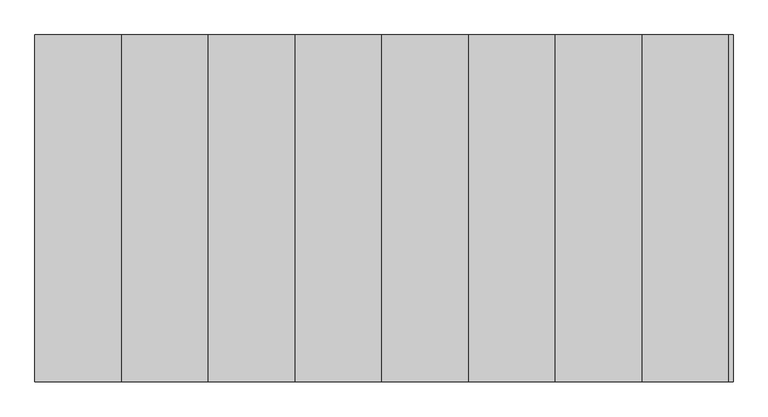
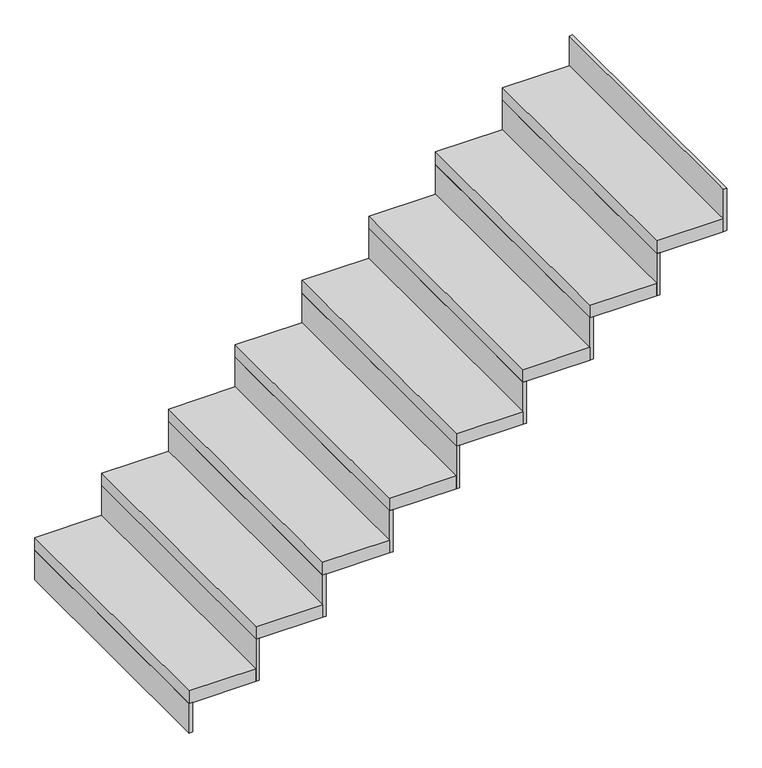
"""IFC4 building model written with IfcOpenShell, lengths in millimetres: stair flight geometry."""

import ifcopenshell
import ifcopenshell.guid

model = None  # the IFC model being written
_history = None  # IfcOwnerHistory: only IFC2X3 demands one
_inside = {}  # id of a spatial element -> (the spatial element, [elements in it])
_under = {}  # id of a project, library or spatial element -> (it, [spatial elements below it])
_declared = {}  # id of a project -> (the project, [libraries it declares])
_typed = {}  # id of a type object -> (the type object, [elements of that type])
_made_of = {}  # id of a material, layer set ... -> (it, [elements and type objects made of it])


def new_model(schema):
    """Start an empty IFC model of exactly this schema.

    Asked for "IFC4X3", IfcOpenShell would pick the latest addendum, in which some entities
    have other attributes; the version numbers below select the first issue.
    IFC2X3 requires an IfcOwnerHistory on every rooted entity: one is made here for all.
    """
    global model, _history
    if schema == "IFC4X3":
        model = ifcopenshell.file(schema_version=(4, 3, 0, 0))
    else:
        model = ifcopenshell.file(schema=schema)
    _inside.clear()
    _under.clear()
    _declared.clear()
    _typed.clear()
    _made_of.clear()
    _history = None
    if model.schema == "IFC2X3":
        org = make("IfcOrganization", Name="unknown")
        user = make(
            "IfcPersonAndOrganization",
            ThePerson=make("IfcPerson", FamilyName="unknown"),
            TheOrganization=org,
        )
        app = make(
            "IfcApplication",
            ApplicationDeveloper=org,
            Version="unknown",
            ApplicationFullName="unknown",
            ApplicationIdentifier="unknown",
        )
        _history = make(
            "IfcOwnerHistory",
            OwningUser=user,
            OwningApplication=app,
            ChangeAction="ADDED",
            CreationDate=0,
        )
    return model


def make(cls, **values):
    """One entity of the class cls with the attributes given. An attribute that is None is left unset."""
    return model.create_entity(
        cls, **{name: value for name, value in values.items() if value is not None}
    )


def rooted(cls, **values):
    """An entity with a GlobalId (a new one), such as an element, a storey or a relation."""
    return make(cls, GlobalId=ifcopenshell.guid.new(), OwnerHistory=_history, **values)


def si_unit(unit_type, name, prefix=None):
    """IfcSIUnit, for example si_unit("LENGTHUNIT", "METRE", prefix="MILLI")."""
    return make("IfcSIUnit", UnitType=unit_type, Prefix=prefix, Name=name)


def assignment(units):
    """IfcUnitAssignment: the units of a project."""
    return None if units is None else make("IfcUnitAssignment", Units=units)


def point(xyz):
    """IfcCartesianPoint."""
    return None if xyz is None else make("IfcCartesianPoint", Coordinates=xyz)


def direction(xyz):
    """IfcDirection."""
    return None if xyz is None else make("IfcDirection", DirectionRatios=xyz)


def frame(location, z_axis=None, x_axis=None):
    """IfcAxis2Placement3D, a coordinate frame: its origin and axes. An axis left out is left unset."""
    return make(
        "IfcAxis2Placement3D",
        Location=point(location),
        Axis=direction(z_axis),
        RefDirection=direction(x_axis),
    )


def origin():
    """The frame at (0, 0, 0) with its axes left unset."""
    return frame((0.0, 0.0, 0.0))


def place(relative_to, where):
    """IfcLocalPlacement: puts the frame where relative to a parent placement (None: the world)."""
    return make(
        "IfcLocalPlacement", PlacementRelTo=relative_to, RelativePlacement=where
    )


def context(
    kind, dimensions, precision=None, world=None, true_north=None, identifier=None
):
    """IfcGeometricRepresentationContext, for example the 3D "Model" context."""
    return make(
        "IfcGeometricRepresentationContext",
        ContextIdentifier=identifier,
        ContextType=kind,
        CoordinateSpaceDimension=dimensions,
        Precision=precision,
        WorldCoordinateSystem=world,
        TrueNorth=true_north,
    )


def project(units=None, contexts=None):
    """IfcProject with its units and contexts."""
    return rooted(
        "IfcProject",
        Name="project",
        RepresentationContexts=contexts,
        UnitsInContext=assignment(units),
    )


def spatial(cls, under=None, at=None, **own):
    """A site, building, storey or space (cls), placed at a placement, below another one or the project."""
    s = rooted(cls, ObjectPlacement=at, **own)
    if under is not None:
        _under.setdefault(under.id(), (under, []))[1].append(s)
    return s


def polyline(points):
    """IfcPolyline through the points."""
    return make("IfcPolyline", Points=[point(p) for p in points])


def outline(outer, holes=None, kind="AREA"):
    """IfcArbitraryClosedProfileDef: a profile drawn as a closed curve; with holes, ...WithVoids."""
    if holes is None:
        return make("IfcArbitraryClosedProfileDef", ProfileType=kind, OuterCurve=outer)
    return make(
        "IfcArbitraryProfileDefWithVoids",
        ProfileType=kind,
        OuterCurve=outer,
        InnerCurves=holes,
    )


def extrude(swept, where, along, depth):
    """IfcExtrudedAreaSolid: the profile swept, set in the frame where, extruded along a direction by depth."""
    return make(
        "IfcExtrudedAreaSolid",
        SweptArea=swept,
        Position=where,
        ExtrudedDirection=direction(along),
        Depth=depth,
    )


def shape(context_of_items, identifier, shape_type, items):
    """IfcShapeRepresentation: the items that make up one representation, for example the "Body"."""
    return make(
        "IfcShapeRepresentation",
        ContextOfItems=context_of_items,
        RepresentationIdentifier=identifier,
        RepresentationType=shape_type,
        Items=items,
    )


def source(mapping_origin, context_of_items, identifier, shape_type, items):
    """IfcRepresentationMap: a shape defined once, which mapped items show again and again."""
    return make(
        "IfcRepresentationMap",
        MappingOrigin=mapping_origin,
        MappedRepresentation=shape(context_of_items, identifier, shape_type, items),
    )


def transform(
    local_origin,
    x_axis=None,
    y_axis=None,
    z_axis=None,
    scale=None,
    scale2=None,
    scale3=None,
    uniform=True,
):
    """IfcCartesianTransformationOperator3D, or its non-uniform kind. x_axis, y_axis, z_axis: its Axis1, 2, 3."""
    if uniform:
        return make(
            "IfcCartesianTransformationOperator3D",
            Axis1=direction(x_axis),
            Axis2=direction(y_axis),
            LocalOrigin=point(local_origin),
            Scale=scale,
            Axis3=direction(z_axis),
        )
    return make(
        "IfcCartesianTransformationOperator3DnonUniform",
        Axis1=direction(x_axis),
        Axis2=direction(y_axis),
        LocalOrigin=point(local_origin),
        Scale=scale,
        Axis3=direction(z_axis),
        Scale2=scale2,
        Scale3=scale3,
    )


def mapped(mapping_source, mapping_target):
    """IfcMappedItem: shows the shape of a source again, moved by a transform."""
    return make(
        "IfcMappedItem", MappingSource=mapping_source, MappingTarget=mapping_target
    )


def made_of(thing, what):
    """Note that an element or type object is made of a material, layer set ...; save() writes the relation."""
    if what is not None:
        _made_of.setdefault(what.id(), (what, []))[1].append(thing)
    return thing


def element(
    cls,
    number,
    at=None,
    inside=None,
    cuts=None,
    type_object=None,
    material=None,
    context=None,
    identifier="Body",
    shape_type=None,
    held_by="IfcProductDefinitionShape",
    body=None,
    shapes=None,
    **own,
):
    """One element of the class cls, such as IfcWall. Its Tag is "e" and its number.

    at: its placement. inside: the storey or other place that contains it. cuts: it is an
    opening in that element (IfcRelVoidsElement). A single representation is given by context,
    identifier, shape_type and body (its items); several are given by shapes. held_by: the class
    of the entity that holds the representations. save() writes the other relations.
    """
    e = rooted(cls, Tag="e%d" % number, ObjectPlacement=at, **own)
    if body is not None:
        shapes = [shape(context, identifier, shape_type, body)]
    if shapes is not None:
        e.Representation = make(held_by, Representations=shapes)
    if inside is not None:
        _inside.setdefault(inside.id(), (inside, []))[1].append(e)
    if cuts is not None:
        rooted(
            "IfcRelVoidsElement", RelatingBuildingElement=cuts, RelatedOpeningElement=e
        )
    if type_object is not None:
        _typed.setdefault(type_object.id(), (type_object, []))[1].append(e)
    return made_of(e, material)


def aggregate(whole, parts):
    """IfcRelAggregates: a whole, such as a stair, and the parts it consists of."""
    return rooted("IfcRelAggregates", RelatingObject=whole, RelatedObjects=parts)


def save(model, path):
    """Write the relations noted so far, then the file.

    IfcRelAggregates (storeys below a building ...), IfcRelContainedInSpatialStructure (elements
    in a storey), IfcRelDefinesByType, IfcRelAssociatesMaterial and IfcRelDeclares: one each for
    every whole, place, type object, material and project.
    """
    for whole, parts in _under.values():
        aggregate(whole, parts)
    for where, things in _inside.values():
        rooted(
            "IfcRelContainedInSpatialStructure",
            RelatedElements=things,
            RelatingStructure=where,
        )
    for kind, things in _typed.values():
        rooted("IfcRelDefinesByType", RelatedObjects=things, RelatingType=kind)
    for what, things in _made_of.values():
        rooted("IfcRelAssociatesMaterial", RelatedObjects=things, RelatingMaterial=what)
    for by, libraries in _declared.values():
        rooted("IfcRelDeclares", RelatingContext=by, RelatedDefinitions=libraries)
    model.write(path)


def stair_flight_022891a7(model_context):
    return source(origin(), model_context, "Body", "SweptSolid", [
        extrude(outline(polyline([(3289.0556606, 2685.7983707), (3276.5556606, 2685.7983707), (3276.5556606, 3685.7983707), (3289.0556606, 3685.7983707), (3289.0556606, 2685.7983707)])), frame((0.0, 0.0, 3300.0), z_axis=(0.0, 0.0, 1.0), x_axis=(1.0, 0.0, 0.0)), (0.0, 0.0, 1.0), 116.6666667),
        extrude(outline(polyline([(3526.5556606, 3685.7983707), (3526.5556606, 2685.7983707), (3276.5556606, 2685.7983707), (3276.5556606, 3685.7983707), (3526.5556606, 3685.7983707)])), frame((0.0, 0.0, 3416.6666667), z_axis=(0.0, 0.0, 1.0), x_axis=(1.0, 0.0, 0.0)), (0.0, 0.0, 1.0), 50.0),
        extrude(outline(polyline([(3539.0556606, 2685.7983707), (3526.5556606, 2685.7983707), (3526.5556606, 3685.7983707), (3539.0556606, 3685.7983707), (3539.0556606, 2685.7983707)])), frame((0.0, 0.0, 3416.6666667), z_axis=(0.0, 0.0, 1.0), x_axis=(1.0, 0.0, 0.0)), (0.0, 0.0, 1.0), 166.6666667),
        extrude(outline(polyline([(3776.5556606, 3685.7983707), (3776.5556606, 2685.7983707), (3526.5556606, 2685.7983707), (3526.5556606, 3685.7983707), (3776.5556606, 3685.7983707)])), frame((0.0, 0.0, 3583.3333333), z_axis=(0.0, 0.0, 1.0), x_axis=(1.0, 0.0, 0.0)), (0.0, 0.0, 1.0), 50.0),
        extrude(outline(polyline([(3789.0556606, 2685.7983707), (3776.5556606, 2685.7983707), (3776.5556606, 3685.7983707), (3789.0556606, 3685.7983707), (3789.0556606, 2685.7983707)])), frame((0.0, 0.0, 3583.3333333), z_axis=(0.0, 0.0, 1.0), x_axis=(1.0, 0.0, 0.0)), (0.0, 0.0, 1.0), 166.6666667),
        extrude(outline(polyline([(4026.5556606, 3685.7983707), (4026.5556606, 2685.7983707), (3776.5556606, 2685.7983707), (3776.5556606, 3685.7983707), (4026.5556606, 3685.7983707)])), frame((0.0, 0.0, 3750.0), z_axis=(0.0, 0.0, 1.0), x_axis=(1.0, 0.0, 0.0)), (0.0, 0.0, 1.0), 50.0),
        extrude(outline(polyline([(4039.0556606, 2685.7983707), (4026.5556606, 2685.7983707), (4026.5556606, 3685.7983707), (4039.0556606, 3685.7983707), (4039.0556606, 2685.7983707)])), frame((0.0, 0.0, 3750.0), z_axis=(0.0, 0.0, 1.0), x_axis=(1.0, 0.0, 0.0)), (0.0, 0.0, 1.0), 166.6666667),
        extrude(outline(polyline([(4276.5556606, 3685.7983707), (4276.5556606, 2685.7983707), (4026.5556606, 2685.7983707), (4026.5556606, 3685.7983707), (4276.5556606, 3685.7983707)])), frame((0.0, 0.0, 3916.6666667), z_axis=(0.0, 0.0, 1.0), x_axis=(1.0, 0.0, 0.0)), (0.0, 0.0, 1.0), 50.0),
        extrude(outline(polyline([(4289.0556606, 2685.7983707), (4276.5556606, 2685.7983707), (4276.5556606, 3685.7983707), (4289.0556606, 3685.7983707), (4289.0556606, 2685.7983707)])), frame((0.0, 0.0, 3916.6666667), z_axis=(0.0, 0.0, 1.0), x_axis=(1.0, 0.0, 0.0)), (0.0, 0.0, 1.0), 166.6666667),
        extrude(outline(polyline([(4526.5556606, 3685.7983707), (4526.5556606, 2685.7983707), (4276.5556606, 2685.7983707), (4276.5556606, 3685.7983707), (4526.5556606, 3685.7983707)])), frame((0.0, 0.0, 4083.3333333), z_axis=(0.0, 0.0, 1.0), x_axis=(1.0, 0.0, 0.0)), (0.0, 0.0, 1.0), 50.0),
        extrude(outline(polyline([(4539.0556606, 2685.7983707), (4526.5556606, 2685.7983707), (4526.5556606, 3685.7983707), (4539.0556606, 3685.7983707), (4539.0556606, 2685.7983707)])), frame((0.0, 0.0, 4083.3333333), z_axis=(0.0, 0.0, 1.0), x_axis=(1.0, 0.0, 0.0)), (0.0, 0.0, 1.0), 166.6666667),
        extrude(outline(polyline([(4776.5556606, 3685.7983707), (4776.5556606, 2685.7983707), (4526.5556606, 2685.7983707), (4526.5556606, 3685.7983707), (4776.5556606, 3685.7983707)])), frame((0.0, 0.0, 4250.0), z_axis=(0.0, 0.0, 1.0), x_axis=(1.0, 0.0, 0.0)), (0.0, 0.0, 1.0), 50.0),
        extrude(outline(polyline([(4789.0556606, 2685.7983707), (4776.5556606, 2685.7983707), (4776.5556606, 3685.7983707), (4789.0556606, 3685.7983707), (4789.0556606, 2685.7983707)])), frame((0.0, 0.0, 4250.0), z_axis=(0.0, 0.0, 1.0), x_axis=(1.0, 0.0, 0.0)), (0.0, 0.0, 1.0), 166.6666667),
        extrude(outline(polyline([(5026.5556606, 3685.7983707), (5026.5556606, 2685.7983707), (4776.5556606, 2685.7983707), (4776.5556606, 3685.7983707), (5026.5556606, 3685.7983707)])), frame((0.0, 0.0, 4416.6666667), z_axis=(0.0, 0.0, 1.0), x_axis=(1.0, 0.0, 0.0)), (0.0, 0.0, 1.0), 50.0),
        extrude(outline(polyline([(5039.0556606, 2685.7983707), (5026.5556606, 2685.7983707), (5026.5556606, 3685.7983707), (5039.0556606, 3685.7983707), (5039.0556606, 2685.7983707)])), frame((0.0, 0.0, 4416.6666667), z_axis=(0.0, 0.0, 1.0), x_axis=(1.0, 0.0, 0.0)), (0.0, 0.0, 1.0), 166.6666667),
        extrude(outline(polyline([(5289.0556606, 2685.7983707), (5276.5556606, 2685.7983707), (5276.5556606, 3685.7983707), (5289.0556606, 3685.7983707), (5289.0556606, 2685.7983707)])), frame((0.0, 0.0, 4583.3333333), z_axis=(0.0, 0.0, 1.0), x_axis=(1.0, 0.0, 0.0)), (0.0, 0.0, 1.0), 166.6666667),
        extrude(outline(polyline([(5276.5556606, 3685.7983707), (5276.5556606, 2685.7983707), (5026.5556606, 2685.7983707), (5026.5556606, 3685.7983707), (5276.5556606, 3685.7983707)])), frame((0.0, 0.0, 4583.3333333), z_axis=(0.0, 0.0, 1.0), x_axis=(1.0, 0.0, 0.0)), (0.0, 0.0, 1.0), 50.0),
    ])


if __name__ == "__main__":
    model = new_model("IFC4")
    model_context = context("Model", 3, world=origin())
    ifc_project = project(units=[si_unit("LENGTHUNIT", "METRE", prefix="MILLI")], contexts=[model_context])
    site = spatial("IfcSite", under=ifc_project)
    building = spatial("IfcBuilding", under=site)
    placement = place(None, origin())
    stair_flight_shape = stair_flight_022891a7(model_context)
    element("IfcStairFlight", 1, at=placement, inside=building, context=model_context, shape_type="MappedRepresentation", body=[
        mapped(stair_flight_shape, transform((0.0, 0.0, 0.0), x_axis=(1.0, 0.0, 0.0), y_axis=(0.0, 1.0, 0.0), z_axis=(0.0, 0.0, 1.0))),
    ])
    save(model, "model.ifc")

# Revit data of these elements
# Project information
#   项目发布日期 = "出图日期"
#   项目状态 = "项目状态"
#   客户姓名 = "所有者"
#   项目地址 = "请在此处输入地址"
#   项目名称 = "项目名称"
#   项目编号 = "项目编号"
